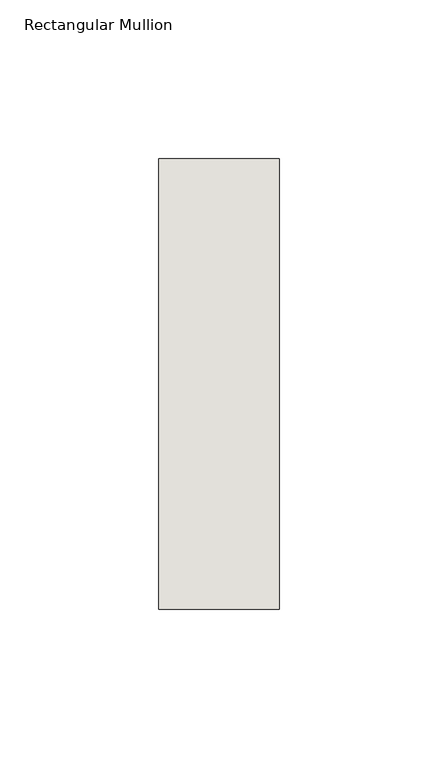
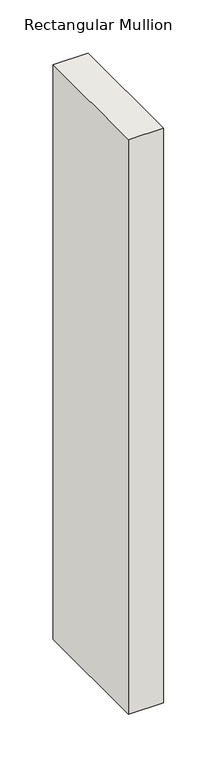
"""IFC4 building model written with IfcOpenShell, lengths in millimetres: wall geometry, Rectangular Mullion : NLRS_21_CWM_hsb-regel 38x142_gen_rsf."""

from ifc_helpers import new_model, si_unit, frame, origin, place, context, project, spatial, polyline, outline, extrude, source, transform, mapped, element, save


def rectangular_mullion_0fff75b4(model_context):
    return source(origin(), model_context, "Body", "SweptSolid", [
        extrude(outline(polyline([(19.0, -71.0), (-19.0, -71.0), (-19.0, 71.0), (19.0, 71.0), (19.0, -71.0)])), frame((0.0, 0.0, -659.0), z_axis=(0.0, 0.0, 1.0), x_axis=(1.0, 0.0, 0.0)), (0.0, 0.0, 1.0), 659.0),
    ])


if __name__ == "__main__":
    model = new_model("IFC4")
    model_context = context("Model", 3, world=origin())
    ifc_project = project(units=[si_unit("LENGTHUNIT", "METRE", prefix="MILLI")], contexts=[model_context])
    site = spatial("IfcSite", under=ifc_project)
    building = spatial("IfcBuilding", under=site)
    placement = place(None, origin())
    rectangular_mullion_shape = rectangular_mullion_0fff75b4(model_context)
    element("IfcWall", 1, ObjectType="Rectangular Mullion : NLRS_21_CWM_hsb-regel 38x142_gen_rsf", at=placement, inside=building, context=model_context, shape_type="MappedRepresentation", body=[
        mapped(rectangular_mullion_shape, transform((0.0, 0.0, 0.0), x_axis=(1.0, 0.0, 0.0), y_axis=(0.0, 1.0, 0.0), z_axis=(0.0, 0.0, 1.0))),
    ])
    save(model, "model.ifc")

# Revit data of these elements
# Type "Rectangular Mullion : NLRS_21_CWM_hsb-regel 38x142_gen_rsf"
#   Type IfcGUID = "07M7mRoiH1CR8m_RSKIwpF"
#   Assembly Code = "21.10"
#   IfcExportAs = "IfcWall"
#   built-in parameter 1007322 = 0.465879 (stored number, unit not read)
#   built-in parameter 1007321 = 0.062336 (stored number, unit not read)
#   built-in parameter 1007320 = 0.062336 (stored number, unit not read)
# Element 1 (IfcWall, "Rectangular Mullion : NLRS_21_CWM_hsb-regel 38x142_gen_rsf")
#   Materials on its faces: "NLRS_i2_hout naaldhout vuren_gen_rsf"
# Materials
#   "NLRS_i2_hout naaldhout vuren_gen_rsf": class "I - Hout", colour RGB 234 199 147, transparency 0, Keynote = "i2", Manufacturer = "Revit Standards Foundation", URL = "www.revitstandards.org", Description = "hout vuren", Cost = 0
